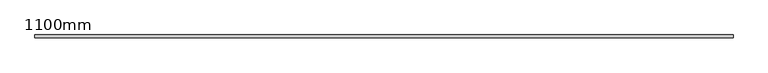
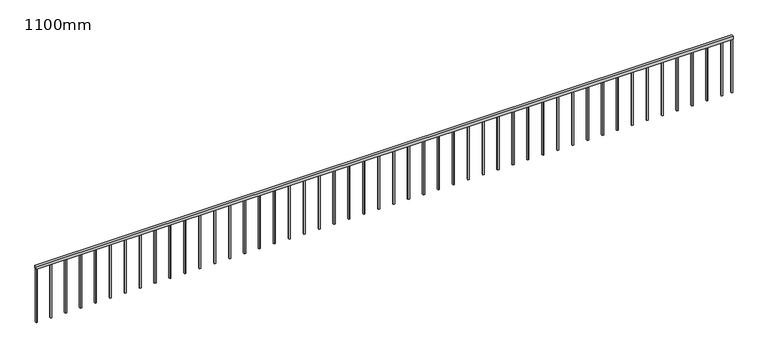
"""IFC4 building model written with IfcOpenShell, lengths in millimetres: railing geometry, 1100mm."""

from ifc_helpers import new_model, si_unit, frame, origin, place, context, project, spatial, polyline, outline, extrude, source, transform, mapped, element, save


def railing_1100mm_35055f6c(model_context):
    return source(origin(), model_context, "Body", "SweptSolid", [
        extrude(outline(polyline([(-21100.0159097, 115.543625), (-21100.0159097, 165.543625), (-8255.7006826, 165.543625), (-8255.7006826, 115.543625), (-21100.0159097, 115.543625)])), frame((0.0, 0.0, 5050.0), z_axis=(0.0, 0.0, 1.0), x_axis=(1.0, 0.0, 0.0)), (0.0, 0.0, 1.0), 50.0),
        extrude(outline(polyline([(-8462.5159097, 153.043625), (-8437.5159097, 153.043625), (-8437.5159097, 128.043625), (-8462.5159097, 128.043625), (-8462.5159097, 153.043625)])), frame((0.0, 0.0, 4000.0), z_axis=(0.0, 0.0, 1.0), x_axis=(1.0, 0.0, 0.0)), (0.0, 0.0, 1.0), 1050.0),
        extrude(outline(polyline([(-8737.5159097, 153.043625), (-8712.5159097, 153.043625), (-8712.5159097, 128.043625), (-8737.5159097, 128.043625), (-8737.5159097, 153.043625)])), frame((0.0, 0.0, 4000.0), z_axis=(0.0, 0.0, 1.0), x_axis=(1.0, 0.0, 0.0)), (0.0, 0.0, 1.0), 1050.0),
        extrude(outline(polyline([(-9012.5159097, 153.043625), (-8987.5159097, 153.043625), (-8987.5159097, 128.043625), (-9012.5159097, 128.043625), (-9012.5159097, 153.043625)])), frame((0.0, 0.0, 4000.0), z_axis=(0.0, 0.0, 1.0), x_axis=(1.0, 0.0, 0.0)), (0.0, 0.0, 1.0), 1050.0),
        extrude(outline(polyline([(-9287.5159097, 153.043625), (-9262.5159097, 153.043625), (-9262.5159097, 128.043625), (-9287.5159097, 128.043625), (-9287.5159097, 153.043625)])), frame((0.0, 0.0, 4000.0), z_axis=(0.0, 0.0, 1.0), x_axis=(1.0, 0.0, 0.0)), (0.0, 0.0, 1.0), 1050.0),
        extrude(outline(polyline([(-9562.5159097, 153.043625), (-9537.5159097, 153.043625), (-9537.5159097, 128.043625), (-9562.5159097, 128.043625), (-9562.5159097, 153.043625)])), frame((0.0, 0.0, 4000.0), z_axis=(0.0, 0.0, 1.0), x_axis=(1.0, 0.0, 0.0)), (0.0, 0.0, 1.0), 1050.0),
        extrude(outline(polyline([(-9837.5159097, 153.043625), (-9812.5159097, 153.043625), (-9812.5159097, 128.043625), (-9837.5159097, 128.043625), (-9837.5159097, 153.043625)])), frame((0.0, 0.0, 4000.0), z_axis=(0.0, 0.0, 1.0), x_axis=(1.0, 0.0, 0.0)), (0.0, 0.0, 1.0), 1050.0),
        extrude(outline(polyline([(-10112.5159097, 153.043625), (-10087.5159097, 153.043625), (-10087.5159097, 128.043625), (-10112.5159097, 128.043625), (-10112.5159097, 153.043625)])), frame((0.0, 0.0, 4000.0), z_axis=(0.0, 0.0, 1.0), x_axis=(1.0, 0.0, 0.0)), (0.0, 0.0, 1.0), 1050.0),
        extrude(outline(polyline([(-10387.5159097, 153.043625), (-10362.5159097, 153.043625), (-10362.5159097, 128.043625), (-10387.5159097, 128.043625), (-10387.5159097, 153.043625)])), frame((0.0, 0.0, 4000.0), z_axis=(0.0, 0.0, 1.0), x_axis=(1.0, 0.0, 0.0)), (0.0, 0.0, 1.0), 1050.0),
        extrude(outline(polyline([(-10662.5159097, 153.043625), (-10637.5159097, 153.043625), (-10637.5159097, 128.043625), (-10662.5159097, 128.043625), (-10662.5159097, 153.043625)])), frame((0.0, 0.0, 4000.0), z_axis=(0.0, 0.0, 1.0), x_axis=(1.0, 0.0, 0.0)), (0.0, 0.0, 1.0), 1050.0),
        extrude(outline(polyline([(-10937.5159097, 153.043625), (-10912.5159097, 153.043625), (-10912.5159097, 128.043625), (-10937.5159097, 128.043625), (-10937.5159097, 153.043625)])), frame((0.0, 0.0, 4000.0), z_axis=(0.0, 0.0, 1.0), x_axis=(1.0, 0.0, 0.0)), (0.0, 0.0, 1.0), 1050.0),
        extrude(outline(polyline([(-11212.5159097, 153.043625), (-11187.5159097, 153.043625), (-11187.5159097, 128.043625), (-11212.5159097, 128.043625), (-11212.5159097, 153.043625)])), frame((0.0, 0.0, 4000.0), z_axis=(0.0, 0.0, 1.0), x_axis=(1.0, 0.0, 0.0)), (0.0, 0.0, 1.0), 1050.0),
        extrude(outline(polyline([(-11487.5159097, 153.043625), (-11462.5159097, 153.043625), (-11462.5159097, 128.043625), (-11487.5159097, 128.043625), (-11487.5159097, 153.043625)])), frame((0.0, 0.0, 4000.0), z_axis=(0.0, 0.0, 1.0), x_axis=(1.0, 0.0, 0.0)), (0.0, 0.0, 1.0), 1050.0),
        extrude(outline(polyline([(-11762.5159097, 153.043625), (-11737.5159097, 153.043625), (-11737.5159097, 128.043625), (-11762.5159097, 128.043625), (-11762.5159097, 153.043625)])), frame((0.0, 0.0, 4000.0), z_axis=(0.0, 0.0, 1.0), x_axis=(1.0, 0.0, 0.0)), (0.0, 0.0, 1.0), 1050.0),
        extrude(outline(polyline([(-12037.5159097, 153.043625), (-12012.5159097, 153.043625), (-12012.5159097, 128.043625), (-12037.5159097, 128.043625), (-12037.5159097, 153.043625)])), frame((0.0, 0.0, 4000.0), z_axis=(0.0, 0.0, 1.0), x_axis=(1.0, 0.0, 0.0)), (0.0, 0.0, 1.0), 1050.0),
        extrude(outline(polyline([(-12312.5159097, 153.043625), (-12287.5159097, 153.043625), (-12287.5159097, 128.043625), (-12312.5159097, 128.043625), (-12312.5159097, 153.043625)])), frame((0.0, 0.0, 4000.0), z_axis=(0.0, 0.0, 1.0), x_axis=(1.0, 0.0, 0.0)), (0.0, 0.0, 1.0), 1050.0),
        extrude(outline(polyline([(-12587.5159097, 153.043625), (-12562.5159097, 153.043625), (-12562.5159097, 128.043625), (-12587.5159097, 128.043625), (-12587.5159097, 153.043625)])), frame((0.0, 0.0, 4000.0), z_axis=(0.0, 0.0, 1.0), x_axis=(1.0, 0.0, 0.0)), (0.0, 0.0, 1.0), 1050.0),
        extrude(outline(polyline([(-12862.5159097, 153.043625), (-12837.5159097, 153.043625), (-12837.5159097, 128.043625), (-12862.5159097, 128.043625), (-12862.5159097, 153.043625)])), frame((0.0, 0.0, 4000.0), z_axis=(0.0, 0.0, 1.0), x_axis=(1.0, 0.0, 0.0)), (0.0, 0.0, 1.0), 1050.0),
        extrude(outline(polyline([(-13137.5159097, 153.043625), (-13112.5159097, 153.043625), (-13112.5159097, 128.043625), (-13137.5159097, 128.043625), (-13137.5159097, 153.043625)])), frame((0.0, 0.0, 4000.0), z_axis=(0.0, 0.0, 1.0), x_axis=(1.0, 0.0, 0.0)), (0.0, 0.0, 1.0), 1050.0),
        extrude(outline(polyline([(-13412.5159097, 153.043625), (-13387.5159097, 153.043625), (-13387.5159097, 128.043625), (-13412.5159097, 128.043625), (-13412.5159097, 153.043625)])), frame((0.0, 0.0, 4000.0), z_axis=(0.0, 0.0, 1.0), x_axis=(1.0, 0.0, 0.0)), (0.0, 0.0, 1.0), 1050.0),
        extrude(outline(polyline([(-13687.5159097, 153.043625), (-13662.5159097, 153.043625), (-13662.5159097, 128.043625), (-13687.5159097, 128.043625), (-13687.5159097, 153.043625)])), frame((0.0, 0.0, 4000.0), z_axis=(0.0, 0.0, 1.0), x_axis=(1.0, 0.0, 0.0)), (0.0, 0.0, 1.0), 1050.0),
        extrude(outline(polyline([(-13962.5159097, 153.043625), (-13937.5159097, 153.043625), (-13937.5159097, 128.043625), (-13962.5159097, 128.043625), (-13962.5159097, 153.043625)])), frame((0.0, 0.0, 4000.0), z_axis=(0.0, 0.0, 1.0), x_axis=(1.0, 0.0, 0.0)), (0.0, 0.0, 1.0), 1050.0),
        extrude(outline(polyline([(-14237.5159097, 153.043625), (-14212.5159097, 153.043625), (-14212.5159097, 128.043625), (-14237.5159097, 128.043625), (-14237.5159097, 153.043625)])), frame((0.0, 0.0, 4000.0), z_axis=(0.0, 0.0, 1.0), x_axis=(1.0, 0.0, 0.0)), (0.0, 0.0, 1.0), 1050.0),
        extrude(outline(polyline([(-14512.5159097, 153.043625), (-14487.5159097, 153.043625), (-14487.5159097, 128.043625), (-14512.5159097, 128.043625), (-14512.5159097, 153.043625)])), frame((0.0, 0.0, 4000.0), z_axis=(0.0, 0.0, 1.0), x_axis=(1.0, 0.0, 0.0)), (0.0, 0.0, 1.0), 1050.0),
        extrude(outline(polyline([(-14787.5159097, 153.043625), (-14762.5159097, 153.043625), (-14762.5159097, 128.043625), (-14787.5159097, 128.043625), (-14787.5159097, 153.043625)])), frame((0.0, 0.0, 4000.0), z_axis=(0.0, 0.0, 1.0), x_axis=(1.0, 0.0, 0.0)), (0.0, 0.0, 1.0), 1050.0),
        extrude(outline(polyline([(-15062.5159097, 153.043625), (-15037.5159097, 153.043625), (-15037.5159097, 128.043625), (-15062.5159097, 128.043625), (-15062.5159097, 153.043625)])), frame((0.0, 0.0, 4000.0), z_axis=(0.0, 0.0, 1.0), x_axis=(1.0, 0.0, 0.0)), (0.0, 0.0, 1.0), 1050.0),
        extrude(outline(polyline([(-15337.5159097, 153.043625), (-15312.5159097, 153.043625), (-15312.5159097, 128.043625), (-15337.5159097, 128.043625), (-15337.5159097, 153.043625)])), frame((0.0, 0.0, 4000.0), z_axis=(0.0, 0.0, 1.0), x_axis=(1.0, 0.0, 0.0)), (0.0, 0.0, 1.0), 1050.0),
        extrude(outline(polyline([(-15612.5159097, 153.043625), (-15587.5159097, 153.043625), (-15587.5159097, 128.043625), (-15612.5159097, 128.043625), (-15612.5159097, 153.043625)])), frame((0.0, 0.0, 4000.0), z_axis=(0.0, 0.0, 1.0), x_axis=(1.0, 0.0, 0.0)), (0.0, 0.0, 1.0), 1050.0),
        extrude(outline(polyline([(-15887.5159097, 153.043625), (-15862.5159097, 153.043625), (-15862.5159097, 128.043625), (-15887.5159097, 128.043625), (-15887.5159097, 153.043625)])), frame((0.0, 0.0, 4000.0), z_axis=(0.0, 0.0, 1.0), x_axis=(1.0, 0.0, 0.0)), (0.0, 0.0, 1.0), 1050.0),
        extrude(outline(polyline([(-16162.5159097, 153.043625), (-16137.5159097, 153.043625), (-16137.5159097, 128.043625), (-16162.5159097, 128.043625), (-16162.5159097, 153.043625)])), frame((0.0, 0.0, 4000.0), z_axis=(0.0, 0.0, 1.0), x_axis=(1.0, 0.0, 0.0)), (0.0, 0.0, 1.0), 1050.0),
        extrude(outline(polyline([(-16437.5159097, 153.043625), (-16412.5159097, 153.043625), (-16412.5159097, 128.043625), (-16437.5159097, 128.043625), (-16437.5159097, 153.043625)])), frame((0.0, 0.0, 4000.0), z_axis=(0.0, 0.0, 1.0), x_axis=(1.0, 0.0, 0.0)), (0.0, 0.0, 1.0), 1050.0),
        extrude(outline(polyline([(-16712.5159097, 153.043625), (-16687.5159097, 153.043625), (-16687.5159097, 128.043625), (-16712.5159097, 128.043625), (-16712.5159097, 153.043625)])), frame((0.0, 0.0, 4000.0), z_axis=(0.0, 0.0, 1.0), x_axis=(1.0, 0.0, 0.0)), (0.0, 0.0, 1.0), 1050.0),
        extrude(outline(polyline([(-16987.5159097, 153.043625), (-16962.5159097, 153.043625), (-16962.5159097, 128.043625), (-16987.5159097, 128.043625), (-16987.5159097, 153.043625)])), frame((0.0, 0.0, 4000.0), z_axis=(0.0, 0.0, 1.0), x_axis=(1.0, 0.0, 0.0)), (0.0, 0.0, 1.0), 1050.0),
        extrude(outline(polyline([(-17262.5159097, 153.043625), (-17237.5159097, 153.043625), (-17237.5159097, 128.043625), (-17262.5159097, 128.043625), (-17262.5159097, 153.043625)])), frame((0.0, 0.0, 4000.0), z_axis=(0.0, 0.0, 1.0), x_axis=(1.0, 0.0, 0.0)), (0.0, 0.0, 1.0), 1050.0),
        extrude(outline(polyline([(-17537.5159097, 153.043625), (-17512.5159097, 153.043625), (-17512.5159097, 128.043625), (-17537.5159097, 128.043625), (-17537.5159097, 153.043625)])), frame((0.0, 0.0, 4000.0), z_axis=(0.0, 0.0, 1.0), x_axis=(1.0, 0.0, 0.0)), (0.0, 0.0, 1.0), 1050.0),
        extrude(outline(polyline([(-17812.5159097, 153.043625), (-17787.5159097, 153.043625), (-17787.5159097, 128.043625), (-17812.5159097, 128.043625), (-17812.5159097, 153.043625)])), frame((0.0, 0.0, 4000.0), z_axis=(0.0, 0.0, 1.0), x_axis=(1.0, 0.0, 0.0)), (0.0, 0.0, 1.0), 1050.0),
        extrude(outline(polyline([(-18087.5159097, 153.043625), (-18062.5159097, 153.043625), (-18062.5159097, 128.043625), (-18087.5159097, 128.043625), (-18087.5159097, 153.043625)])), frame((0.0, 0.0, 4000.0), z_axis=(0.0, 0.0, 1.0), x_axis=(1.0, 0.0, 0.0)), (0.0, 0.0, 1.0), 1050.0),
        extrude(outline(polyline([(-18362.5159097, 153.043625), (-18337.5159097, 153.043625), (-18337.5159097, 128.043625), (-18362.5159097, 128.043625), (-18362.5159097, 153.043625)])), frame((0.0, 0.0, 4000.0), z_axis=(0.0, 0.0, 1.0), x_axis=(1.0, 0.0, 0.0)), (0.0, 0.0, 1.0), 1050.0),
        extrude(outline(polyline([(-18637.5159097, 153.043625), (-18612.5159097, 153.043625), (-18612.5159097, 128.043625), (-18637.5159097, 128.043625), (-18637.5159097, 153.043625)])), frame((0.0, 0.0, 4000.0), z_axis=(0.0, 0.0, 1.0), x_axis=(1.0, 0.0, 0.0)), (0.0, 0.0, 1.0), 1050.0),
        extrude(outline(polyline([(-18912.5159097, 153.043625), (-18887.5159097, 153.043625), (-18887.5159097, 128.043625), (-18912.5159097, 128.043625), (-18912.5159097, 153.043625)])), frame((0.0, 0.0, 4000.0), z_axis=(0.0, 0.0, 1.0), x_axis=(1.0, 0.0, 0.0)), (0.0, 0.0, 1.0), 1050.0),
        extrude(outline(polyline([(-19187.5159097, 153.043625), (-19162.5159097, 153.043625), (-19162.5159097, 128.043625), (-19187.5159097, 128.043625), (-19187.5159097, 153.043625)])), frame((0.0, 0.0, 4000.0), z_axis=(0.0, 0.0, 1.0), x_axis=(1.0, 0.0, 0.0)), (0.0, 0.0, 1.0), 1050.0),
        extrude(outline(polyline([(-19462.5159097, 153.043625), (-19437.5159097, 153.043625), (-19437.5159097, 128.043625), (-19462.5159097, 128.043625), (-19462.5159097, 153.043625)])), frame((0.0, 0.0, 4000.0), z_axis=(0.0, 0.0, 1.0), x_axis=(1.0, 0.0, 0.0)), (0.0, 0.0, 1.0), 1050.0),
        extrude(outline(polyline([(-19737.5159097, 153.043625), (-19712.5159097, 153.043625), (-19712.5159097, 128.043625), (-19737.5159097, 128.043625), (-19737.5159097, 153.043625)])), frame((0.0, 0.0, 4000.0), z_axis=(0.0, 0.0, 1.0), x_axis=(1.0, 0.0, 0.0)), (0.0, 0.0, 1.0), 1050.0),
        extrude(outline(polyline([(-20012.5159097, 153.043625), (-19987.5159097, 153.043625), (-19987.5159097, 128.043625), (-20012.5159097, 128.043625), (-20012.5159097, 153.043625)])), frame((0.0, 0.0, 4000.0), z_axis=(0.0, 0.0, 1.0), x_axis=(1.0, 0.0, 0.0)), (0.0, 0.0, 1.0), 1050.0),
        extrude(outline(polyline([(-20287.5159097, 153.043625), (-20262.5159097, 153.043625), (-20262.5159097, 128.043625), (-20287.5159097, 128.043625), (-20287.5159097, 153.043625)])), frame((0.0, 0.0, 4000.0), z_axis=(0.0, 0.0, 1.0), x_axis=(1.0, 0.0, 0.0)), (0.0, 0.0, 1.0), 1050.0),
        extrude(outline(polyline([(-20562.5159097, 153.043625), (-20537.5159097, 153.043625), (-20537.5159097, 128.043625), (-20562.5159097, 128.043625), (-20562.5159097, 153.043625)])), frame((0.0, 0.0, 4000.0), z_axis=(0.0, 0.0, 1.0), x_axis=(1.0, 0.0, 0.0)), (0.0, 0.0, 1.0), 1050.0),
        extrude(outline(polyline([(-20837.5159097, 153.043625), (-20812.5159097, 153.043625), (-20812.5159097, 128.043625), (-20837.5159097, 128.043625), (-20837.5159097, 153.043625)])), frame((0.0, 0.0, 4000.0), z_axis=(0.0, 0.0, 1.0), x_axis=(1.0, 0.0, 0.0)), (0.0, 0.0, 1.0), 1050.0),
        extrude(outline(polyline([(-8280.7006826, 153.043625), (-8255.7006826, 153.043625), (-8255.7006826, 128.043625), (-8280.7006826, 128.043625), (-8280.7006826, 153.043625)])), frame((0.0, 0.0, 4000.0), z_axis=(0.0, 0.0, 1.0), x_axis=(1.0, 0.0, 0.0)), (0.0, 0.0, 1.0), 1050.0),
        extrude(outline(polyline([(-21100.0159097, 153.043625), (-21075.0159097, 153.043625), (-21075.0159097, 128.043625), (-21100.0159097, 128.043625), (-21100.0159097, 153.043625)])), frame((0.0, 0.0, 4000.0), z_axis=(0.0, 0.0, 1.0), x_axis=(1.0, 0.0, 0.0)), (0.0, 0.0, 1.0), 1050.0),
    ])


if __name__ == "__main__":
    model = new_model("IFC4")
    model_context = context("Model", 3, world=origin())
    ifc_project = project(units=[si_unit("LENGTHUNIT", "METRE", prefix="MILLI")], contexts=[model_context])
    site = spatial("IfcSite", under=ifc_project)
    building = spatial("IfcBuilding", under=site)
    placement = place(None, origin())
    railing_1100mm_shape = railing_1100mm_35055f6c(model_context)
    element("IfcRailing", 1, ObjectType="1100mm", at=placement, inside=building, context=model_context, shape_type="MappedRepresentation", body=[
        mapped(railing_1100mm_shape, transform((0.0, 0.0, 0.0), x_axis=(1.0, 0.0, 0.0), y_axis=(0.0, 1.0, 0.0), z_axis=(0.0, 0.0, 1.0))),
    ])
    save(model, "model.ifc")
